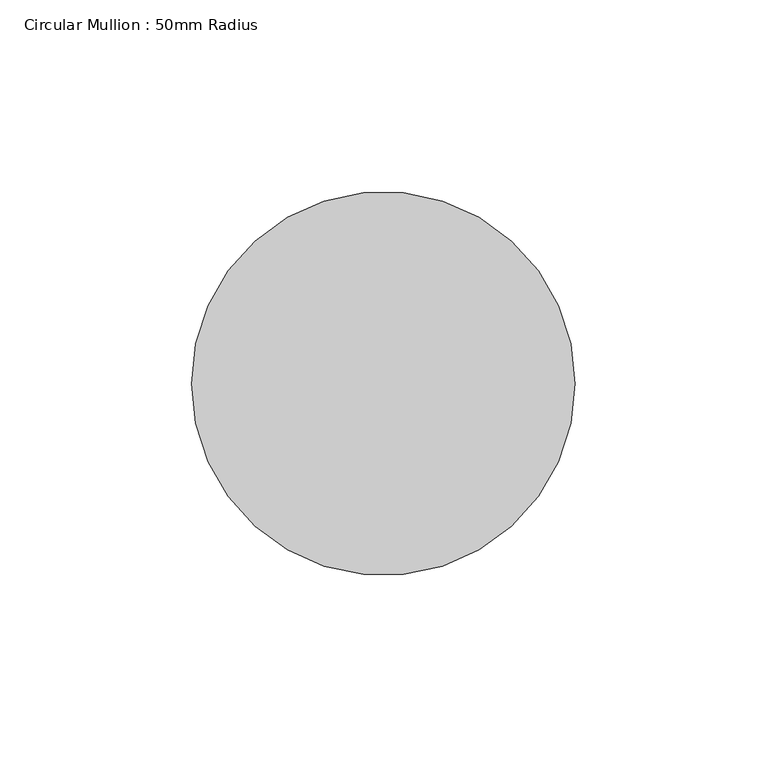
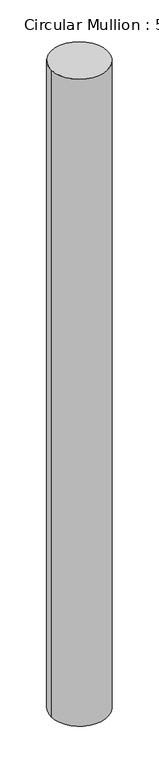
"""IFC4 building model written with IfcOpenShell, lengths in millimetres: member geometry, Circular Mullion : 50mm Radius."""

from ifc_helpers import new_model, si_unit, point, frame, origin, origin_2d, place, context, project, spatial, circle_curve, trimmed, segment, composite_curve, outline, extrude, source, transform, mapped, element, save


def circular_mullion_50mm_radius_634924c6(model_context):
    return source(origin(), model_context, "Body", "SweptSolid", [
        extrude(outline(composite_curve([segment(trimmed(circle_curve(origin_2d(), 50.0), [point((50.0, 0.0))], [point((-50.0, 0.0))], False, "CARTESIAN"), True, "CONTINUOUS"), segment(trimmed(circle_curve(origin_2d(), 50.0), [point((-50.0, 0.0))], [point((50.0, 0.0))], False, "CARTESIAN"), True, "CONTINUOUS")], self_intersect=False)), frame((0.0, 0.0, -1207.4793819), z_axis=(0.0, 0.0, 1.0), x_axis=(1.0, 0.0, 0.0)), (0.0, 0.0, 1.0), 1207.4793819),
    ])


if __name__ == "__main__":
    model = new_model("IFC4")
    model_context = context("Model", 3, world=origin())
    ifc_project = project(units=[si_unit("LENGTHUNIT", "METRE", prefix="MILLI")], contexts=[model_context])
    site = spatial("IfcSite", under=ifc_project)
    building = spatial("IfcBuilding", under=site)
    placement = place(None, origin())
    circular_mullion_50mm_radius_shape = circular_mullion_50mm_radius_634924c6(model_context)
    element("IfcMember", 1, ObjectType="Circular Mullion : 50mm Radius", at=placement, inside=building, context=model_context, shape_type="MappedRepresentation", body=[
        mapped(circular_mullion_50mm_radius_shape, transform((0.0, 0.0, 0.0), x_axis=(1.0, 0.0, 0.0), y_axis=(0.0, 1.0, 0.0), z_axis=(0.0, 0.0, 1.0))),
    ])
    save(model, "model.ifc")

# Revit data of these elements
# Type "Circular Mullion : 50mm Radius"
#   built-in parameter 1007350 = 0.164042 (stored number, unit not read)
# Element 1 (IfcMember, "Circular Mullion : 50mm Radius")
#   Materials on its faces: "Aluminium"
# Materials
#   "Aluminium": class "Metal", colour RGB 247 247 247, transparency 0, Description = "Aluminium 6061", Cost = 0
